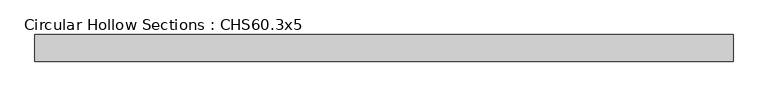
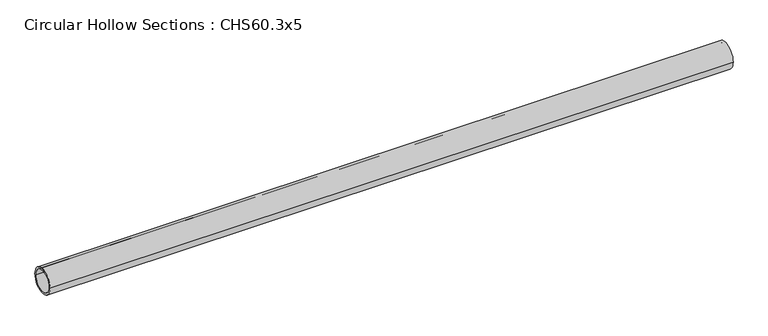
"""IFC4 building model written with IfcOpenShell, lengths in millimetres: beam geometry, Circular Hollow Sections : CHS60.3x5."""

from ifc_helpers import new_model, si_unit, point, frame, origin, origin_2d, place, context, project, spatial, circle_curve, trimmed, segment, composite_curve, outline, extrude, source, transform, mapped, element, save


def circular_hollow_sections_chs60_3x5_b8a643cb(model_context):
    return source(origin(), model_context, "Body", "SweptSolid", [
        extrude(outline(composite_curve([segment(trimmed(circle_curve(origin_2d(), 30.15), [point((-30.15, 0.0))], [point((30.15, 0.0))], False, "CARTESIAN"), True, "CONTINUOUS"), segment(trimmed(circle_curve(origin_2d(), 30.15), [point((30.15, 0.0))], [point((-30.15, 0.0))], False, "CARTESIAN"), True, "CONTINUOUS")], self_intersect=False), holes=[composite_curve([segment(trimmed(circle_curve(origin_2d(), 25.15), [point((25.15, 0.0))], [point((-25.15, 0.0))], True, "CARTESIAN"), True, "CONTINUOUS"), segment(trimmed(circle_curve(origin_2d(), 25.15), [point((-25.15, 0.0))], [point((25.15, 0.0))], True, "CARTESIAN"), True, "CONTINUOUS")], self_intersect=False)]), frame((-790.0, 0.0, 0.0), z_axis=(1.0, 0.0, 0.0), x_axis=(0.0, 1.0, 0.0)), (0.0, 0.0, 1.0), 1580.0),
    ])


if __name__ == "__main__":
    model = new_model("IFC4")
    model_context = context("Model", 3, world=origin())
    ifc_project = project(units=[si_unit("LENGTHUNIT", "METRE", prefix="MILLI")], contexts=[model_context])
    site = spatial("IfcSite", under=ifc_project)
    building = spatial("IfcBuilding", under=site)
    placement = place(None, origin())
    circular_hollow_sections_chs60_3x5_shape = circular_hollow_sections_chs60_3x5_b8a643cb(model_context)
    element("IfcBeam", 1, ObjectType="Circular Hollow Sections : CHS60.3x5", at=placement, inside=building, context=model_context, shape_type="MappedRepresentation", body=[
        mapped(circular_hollow_sections_chs60_3x5_shape, transform((0.0, 0.0, 0.0), x_axis=(1.0, 0.0, 0.0), y_axis=(0.0, 1.0, 0.0), z_axis=(0.0, 0.0, 1.0))),
    ])
    save(model, "model.ifc")

# Revit data of these elements
# Type "Circular Hollow Sections : CHS60.3x5"
#   Description = "Hollow Core Steel Roof Truss Member"
#   Type Comments = "Steel 50-355"
#   Assembly Code = "F10"
#   t = 5 mm
#   W = 0.00682
#   Start Extension Calculation [instance default] = 3000 mm
#   Start Extension [instance default] = -12.7 mm
#   Length [instance default] = 1500 mm
#   OD = 60.3 mm
#   End Extension Calculation [instance default] = 3000 mm
#   End Extension [instance default] = -12.7 mm
#   A = 0.000869 m²
#   Structural Material [instance default] = Metal - Steel 50-355
# Element 1 (IfcBeam, "Circular Hollow Sections : CHS60.3x5")
#   Materials on its faces: "Metal - Steel 50-355"
# Materials
#   "Metal - Steel 50-355": class "Metal", colour RGB 247 247 247, transparency 0
